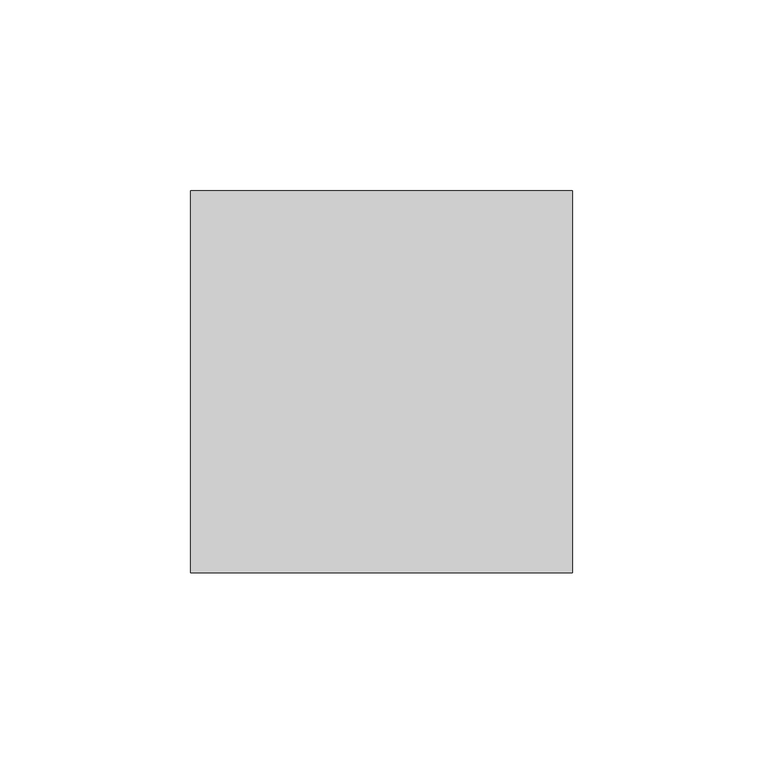
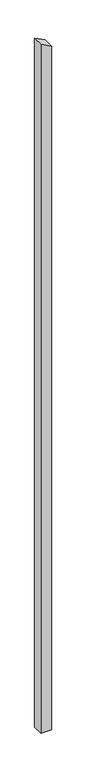
"""IFC4 building model written with IfcOpenShell, lengths in millimetres: column geometry, Holzstütze 159406 : Holzstütze 159406."""

from ifc_helpers import new_model, si_unit, frame, origin, place, context, project, spatial, polyline, outline, extrude, source, transform, mapped, element, save


def column_ac924ca4(model_context):
    return source(origin(), model_context, "Body", "SweptSolid", [
        extrude(outline(polyline([(-500.0, 174197.7593015), (-500.0, 174297.7593015), (6345.7118258, 174297.7593015), (6396.6643707, 174197.7593015), (-500.0, 174197.7593015)])), frame((0.0, 44151.7297978, 0.0), z_axis=(0.0, 1.0, 0.0), x_axis=(0.0, 0.0, 1.0)), (0.0, 0.0, 1.0), 100.0),
    ])


if __name__ == "__main__":
    model = new_model("IFC4")
    model_context = context("Model", 3, world=origin())
    ifc_project = project(units=[si_unit("LENGTHUNIT", "METRE", prefix="MILLI")], contexts=[model_context])
    site = spatial("IfcSite", under=ifc_project)
    building = spatial("IfcBuilding", under=site)
    placement = place(None, origin())
    column_shape = column_ac924ca4(model_context)
    element("IfcColumn", 1, ObjectType="Holzstütze 159406 : Holzstütze 159406", at=placement, inside=building, context=model_context, shape_type="MappedRepresentation", body=[
        mapped(column_shape, transform((0.0, 0.0, 0.0), x_axis=(1.0, 0.0, 0.0), y_axis=(0.0, 1.0, 0.0), z_axis=(0.0, 0.0, 1.0))),
    ])
    save(model, "model.ifc")

# Revit data of these elements
# Type "Holzstütze 159406 : Holzstütze 159406"
#   Abrechnungsart = "m"
#   Allright_Bauteil_ID = "0152St 0000143354"
#   Bezeichnung = "Holzstütze"
#   Codetext = "ST-HOLZ\\"
#   Gewerk = "Zimmer- und Holzbauarbeiten"
#   Material = "Holz"
#   Objektname = "Stütze"
#   NameOverride = "Holzstütze"
#   Reference = "Holzstütze"
#   Status = "NEW"
#   ThermalTransmittance = 0.0000 BTU/(h·ft²·°F)
#   Roll = 0.00°
#   Slope = 0.00°
#   2D Interaktion = yes
#   IsExternal = yes
#   LoadBearing = yes
# Element 1 (IfcColumn, "Holzstütze 159406 : Holzstütze 159406")
#   Materials on its faces: "holzschalung"
# Materials
#   "holzschalung": class "Unassigned", colour RGB 128 128 128, transparency 0
